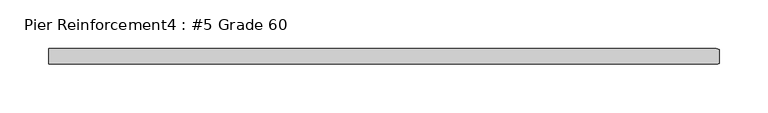
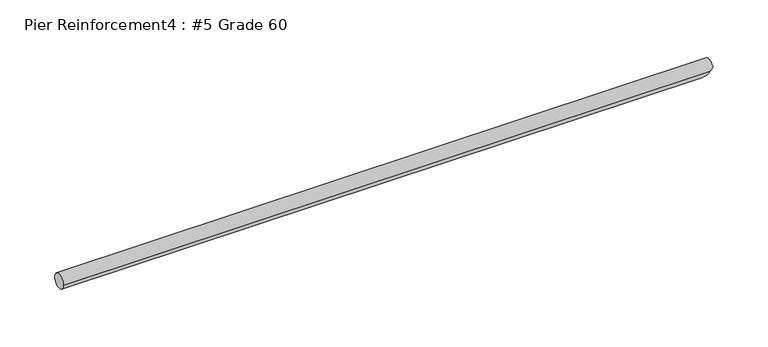
"""IFC4 building model written with IfcOpenShell, lengths in millimetres: proxy geometry, Pier Reinforcement4 : #5 Grade 60."""

import ifcopenshell
import ifcopenshell.guid

model = None  # the IFC model being written
_history = None  # IfcOwnerHistory: only IFC2X3 demands one
_inside = {}  # id of a spatial element -> (the spatial element, [elements in it])
_under = {}  # id of a project, library or spatial element -> (it, [spatial elements below it])
_declared = {}  # id of a project -> (the project, [libraries it declares])
_typed = {}  # id of a type object -> (the type object, [elements of that type])
_made_of = {}  # id of a material, layer set ... -> (it, [elements and type objects made of it])


def new_model(schema):
    """Start an empty IFC model of exactly this schema.

    Asked for "IFC4X3", IfcOpenShell would pick the latest addendum, in which some entities
    have other attributes; the version numbers below select the first issue.
    IFC2X3 requires an IfcOwnerHistory on every rooted entity: one is made here for all.
    """
    global model, _history
    if schema == "IFC4X3":
        model = ifcopenshell.file(schema_version=(4, 3, 0, 0))
    else:
        model = ifcopenshell.file(schema=schema)
    _inside.clear()
    _under.clear()
    _declared.clear()
    _typed.clear()
    _made_of.clear()
    _history = None
    if model.schema == "IFC2X3":
        org = make("IfcOrganization", Name="unknown")
        user = make(
            "IfcPersonAndOrganization",
            ThePerson=make("IfcPerson", FamilyName="unknown"),
            TheOrganization=org,
        )
        app = make(
            "IfcApplication",
            ApplicationDeveloper=org,
            Version="unknown",
            ApplicationFullName="unknown",
            ApplicationIdentifier="unknown",
        )
        _history = make(
            "IfcOwnerHistory",
            OwningUser=user,
            OwningApplication=app,
            ChangeAction="ADDED",
            CreationDate=0,
        )
    return model


def make(cls, **values):
    """One entity of the class cls with the attributes given. An attribute that is None is left unset."""
    return model.create_entity(
        cls, **{name: value for name, value in values.items() if value is not None}
    )


def rooted(cls, **values):
    """An entity with a GlobalId (a new one), such as an element, a storey or a relation."""
    return make(cls, GlobalId=ifcopenshell.guid.new(), OwnerHistory=_history, **values)


def si_unit(unit_type, name, prefix=None):
    """IfcSIUnit, for example si_unit("LENGTHUNIT", "METRE", prefix="MILLI")."""
    return make("IfcSIUnit", UnitType=unit_type, Prefix=prefix, Name=name)


def assignment(units):
    """IfcUnitAssignment: the units of a project."""
    return None if units is None else make("IfcUnitAssignment", Units=units)


def point(xyz):
    """IfcCartesianPoint."""
    return None if xyz is None else make("IfcCartesianPoint", Coordinates=xyz)


def direction(xyz):
    """IfcDirection."""
    return None if xyz is None else make("IfcDirection", DirectionRatios=xyz)


def frame(location, z_axis=None, x_axis=None):
    """IfcAxis2Placement3D, a coordinate frame: its origin and axes. An axis left out is left unset."""
    return make(
        "IfcAxis2Placement3D",
        Location=point(location),
        Axis=direction(z_axis),
        RefDirection=direction(x_axis),
    )


def origin():
    """The frame at (0, 0, 0) with its axes left unset."""
    return frame((0.0, 0.0, 0.0))


def place(relative_to, where):
    """IfcLocalPlacement: puts the frame where relative to a parent placement (None: the world)."""
    return make(
        "IfcLocalPlacement", PlacementRelTo=relative_to, RelativePlacement=where
    )


def context(
    kind, dimensions, precision=None, world=None, true_north=None, identifier=None
):
    """IfcGeometricRepresentationContext, for example the 3D "Model" context."""
    return make(
        "IfcGeometricRepresentationContext",
        ContextIdentifier=identifier,
        ContextType=kind,
        CoordinateSpaceDimension=dimensions,
        Precision=precision,
        WorldCoordinateSystem=world,
        TrueNorth=true_north,
    )


def project(units=None, contexts=None):
    """IfcProject with its units and contexts."""
    return rooted(
        "IfcProject",
        Name="project",
        RepresentationContexts=contexts,
        UnitsInContext=assignment(units),
    )


def spatial(cls, under=None, at=None, **own):
    """A site, building, storey or space (cls), placed at a placement, below another one or the project."""
    s = rooted(cls, ObjectPlacement=at, **own)
    if under is not None:
        _under.setdefault(under.id(), (under, []))[1].append(s)
    return s


def circle_curve(where, radius):
    """IfcCircle in the frame where."""
    return make("IfcCircle", Position=where, Radius=radius)


def ellipse_curve(where, semi_axis1, semi_axis2):
    """IfcEllipse in the frame where."""
    return make(
        "IfcEllipse", Position=where, SemiAxis1=semi_axis1, SemiAxis2=semi_axis2
    )


def shape(context_of_items, identifier, shape_type, items):
    """IfcShapeRepresentation: the items that make up one representation, for example the "Body"."""
    return make(
        "IfcShapeRepresentation",
        ContextOfItems=context_of_items,
        RepresentationIdentifier=identifier,
        RepresentationType=shape_type,
        Items=items,
    )


def source(mapping_origin, context_of_items, identifier, shape_type, items):
    """IfcRepresentationMap: a shape defined once, which mapped items show again and again."""
    return make(
        "IfcRepresentationMap",
        MappingOrigin=mapping_origin,
        MappedRepresentation=shape(context_of_items, identifier, shape_type, items),
    )


def transform(
    local_origin,
    x_axis=None,
    y_axis=None,
    z_axis=None,
    scale=None,
    scale2=None,
    scale3=None,
    uniform=True,
):
    """IfcCartesianTransformationOperator3D, or its non-uniform kind. x_axis, y_axis, z_axis: its Axis1, 2, 3."""
    if uniform:
        return make(
            "IfcCartesianTransformationOperator3D",
            Axis1=direction(x_axis),
            Axis2=direction(y_axis),
            LocalOrigin=point(local_origin),
            Scale=scale,
            Axis3=direction(z_axis),
        )
    return make(
        "IfcCartesianTransformationOperator3DnonUniform",
        Axis1=direction(x_axis),
        Axis2=direction(y_axis),
        LocalOrigin=point(local_origin),
        Scale=scale,
        Axis3=direction(z_axis),
        Scale2=scale2,
        Scale3=scale3,
    )


def mapped(mapping_source, mapping_target):
    """IfcMappedItem: shows the shape of a source again, moved by a transform."""
    return make(
        "IfcMappedItem", MappingSource=mapping_source, MappingTarget=mapping_target
    )


def made_of(thing, what):
    """Note that an element or type object is made of a material, layer set ...; save() writes the relation."""
    if what is not None:
        _made_of.setdefault(what.id(), (what, []))[1].append(thing)
    return thing


def element(
    cls,
    number,
    at=None,
    inside=None,
    cuts=None,
    type_object=None,
    material=None,
    context=None,
    identifier="Body",
    shape_type=None,
    held_by="IfcProductDefinitionShape",
    body=None,
    shapes=None,
    **own,
):
    """One element of the class cls, such as IfcWall. Its Tag is "e" and its number.

    at: its placement. inside: the storey or other place that contains it. cuts: it is an
    opening in that element (IfcRelVoidsElement). A single representation is given by context,
    identifier, shape_type and body (its items); several are given by shapes. held_by: the class
    of the entity that holds the representations. save() writes the other relations.
    """
    e = rooted(cls, Tag="e%d" % number, ObjectPlacement=at, **own)
    if body is not None:
        shapes = [shape(context, identifier, shape_type, body)]
    if shapes is not None:
        e.Representation = make(held_by, Representations=shapes)
    if inside is not None:
        _inside.setdefault(inside.id(), (inside, []))[1].append(e)
    if cuts is not None:
        rooted(
            "IfcRelVoidsElement", RelatingBuildingElement=cuts, RelatedOpeningElement=e
        )
    if type_object is not None:
        _typed.setdefault(type_object.id(), (type_object, []))[1].append(e)
    return made_of(e, material)


def aggregate(whole, parts):
    """IfcRelAggregates: a whole, such as a stair, and the parts it consists of."""
    return rooted("IfcRelAggregates", RelatingObject=whole, RelatedObjects=parts)


def save(model, path):
    """Write the relations noted so far, then the file.

    IfcRelAggregates (storeys below a building ...), IfcRelContainedInSpatialStructure (elements
    in a storey), IfcRelDefinesByType, IfcRelAssociatesMaterial and IfcRelDeclares: one each for
    every whole, place, type object, material and project.
    """
    for whole, parts in _under.values():
        aggregate(whole, parts)
    for where, things in _inside.values():
        rooted(
            "IfcRelContainedInSpatialStructure",
            RelatedElements=things,
            RelatingStructure=where,
        )
    for kind, things in _typed.values():
        rooted("IfcRelDefinesByType", RelatedObjects=things, RelatingType=kind)
    for what, things in _made_of.values():
        rooted("IfcRelAssociatesMaterial", RelatedObjects=things, RelatingMaterial=what)
    for by, libraries in _declared.values():
        rooted("IfcRelDeclares", RelatingContext=by, RelatedDefinitions=libraries)
    model.write(path)


def plane_surface(at):
    """IfcPlane: the flat surface through the origin of the frame at, square to its z axis."""
    return make("IfcPlane", Position=at)


def cylinder_surface(at, radius):
    """IfcCylindricalSurface: all points at the distance radius from the z axis of the frame at."""
    return make("IfcCylindricalSurface", Position=at, Radius=radius)


def advanced_brep(points, edges, surfaces, faces):
    """IfcAdvancedBrep: a solid bounded by faces that lie on surfaces and meet in shared edges.

    An edge is (start, end): straight between two places in points (the first is 0);
    or (start, end, curve); or (start, end, curve, False) where it runs against its curve.
    A face is (place in surfaces, loops), or (place, loops, False) where it looks against
    its surface's normal. A loop lists edges by number (the first is 1), with a minus sign
    where the edge is run from its end to its start. The first loop is the outer one.
    """
    corners = [point(p) for p in points]
    vertices = [make("IfcVertexPoint", VertexGeometry=c) for c in corners]
    made = []
    for start, end, *more in edges:
        made.append(
            make(
                "IfcEdgeCurve",
                EdgeStart=vertices[start],
                EdgeEnd=vertices[end],
                EdgeGeometry=more[0] if more else make("IfcPolyline", Points=[corners[start], corners[end]]),
                SameSense=more[1] if len(more) > 1 else True,
            )
        )
    hull = []
    for where, loops, *sense in faces:
        bounds = []
        for j, loop in enumerate(loops):
            ring = [make("IfcOrientedEdge", EdgeElement=made[abs(k) - 1], Orientation=k > 0) for k in loop]
            bounds.append(
                make(
                    "IfcFaceOuterBound" if j == 0 else "IfcFaceBound",
                    Bound=make("IfcEdgeLoop", EdgeList=ring),
                    Orientation=True,
                )
            )
        hull.append(make("IfcAdvancedFace", Bounds=bounds, FaceSurface=surfaces[where], SameSense=sense[0] if sense else True))
    return make("IfcAdvancedBrep", Outer=make("IfcClosedShell", CfsFaces=hull))


def pier_reinforcement4_5_grade_60_3385e020(model_context):
    return source(origin(), model_context, "Body", "AdvancedBrep", [
        advanced_brep(
        [(590233.9922365, -534089.3915452, -52.3875), (590233.9922365, -534103.941223, -52.3875), (589548.1922365, -534088.7288841, -55.5625), (589548.1922365, -534104.6038841, -55.5625), (590230.8172365, -534104.6038841, -55.5625), (590230.8172365, -534088.7288841, -55.5625), (590222.8797365, -534096.6663841, -63.5)],
        [
            (0, 1, circle_curve(frame((590233.9922365, -534096.6663841, -55.5625), z_axis=(1.0, 0.0, 0.0), x_axis=(0.0, -1.0, 0.0)), 7.9375)),
            (1, 0),
            (2, 3, circle_curve(frame((589548.1922365, -534096.6663841, -55.5625), z_axis=(-1.0, 0.0, 0.0), x_axis=(0.0, -1.0, 0.0)), 7.9375)),
            (3, 2, circle_curve(frame((589548.1922365, -534096.6663841, -55.5625), z_axis=(-1.0, 0.0, 0.0), x_axis=(0.0, -1.0, 0.0)), 7.9375)),
            (3, 4),
            (4, 1, ellipse_curve(frame((590230.8172365, -534096.6663841, -55.5625), z_axis=(-0.7071067811865462, 0.0, 0.7071067811865489), x_axis=(0.7071067811865487, 0.0, 0.7071067811865462)), 11.2253202, 7.9375)),
            (0, 5, ellipse_curve(frame((590230.8172365, -534096.6663841, -55.5625), z_axis=(-0.7071067811865462, 0.0, 0.7071067811865489), x_axis=(0.7071067811865487, 0.0, 0.7071067811865462)), 11.2253202, 7.9375)),
            (5, 2),
            (5, 6, ellipse_curve(frame((590230.8172365, -534096.6663841, -55.5625), z_axis=(-0.7071067811865462, 0.0, 0.7071067811865489), x_axis=(0.7071067811865487, 0.0, 0.7071067811865462)), 11.2253202, 7.9375)),
            (6, 4, ellipse_curve(frame((590230.8172365, -534096.6663841, -55.5625), z_axis=(-0.7071067811865462, 0.0, 0.7071067811865489), x_axis=(0.7071067811865487, 0.0, 0.7071067811865462)), 11.2253202, 7.9375)),
        ],
        [
            plane_surface(frame((590233.9922365, -534104.6038841, -55.5625), z_axis=(1.0, 0.0, 0.0), x_axis=(0.0, 0.0, -1.0))),
            plane_surface(frame((589548.1922365, -534104.6038841, -55.5625), z_axis=(-1.0, 0.0, 0.0), x_axis=(0.0, 0.0, 1.0))),
            cylinder_surface(frame((589548.1922365, -534096.6663841, -55.5625), z_axis=(1.0, 0.0, 0.0), x_axis=(0.0, -1.0, 0.0)), 7.9375),
            plane_surface(frame((590222.8797365, -534128.4163841, -63.5), z_axis=(0.7071067811865462, 0.0, -0.7071067811865489), x_axis=(0.0, 1.0, 0.0))),
        ],
        [
            (0, [[1, 2]]),
            (1, [[3, 4]]),
            (2, [[-4, 5, 6, -1, 7, 8]]),
            (2, [[-3, -8, 9, 10, -5]]),
            (3, [[-2, -6, -10, -9, -7]]),
        ],
    ),
    ])


if __name__ == "__main__":
    model = new_model("IFC4")
    model_context = context("Model", 3, world=origin())
    ifc_project = project(units=[si_unit("LENGTHUNIT", "METRE", prefix="MILLI")], contexts=[model_context])
    site = spatial("IfcSite", under=ifc_project)
    building = spatial("IfcBuilding", under=site)
    placement = place(None, origin())
    pier_reinforcement4_5_grade_60_shape = pier_reinforcement4_5_grade_60_3385e020(model_context)
    element("IfcBuildingElementProxy", 1, Name="Pier Reinforcement4 : #5 Grade 60", ObjectType="Pier Reinforcement4 : #5 Grade 60", at=placement, inside=building, context=model_context, shape_type="MappedRepresentation", body=[
        mapped(pier_reinforcement4_5_grade_60_shape, transform((0.0, 0.0, 0.0), x_axis=(1.0, 0.0, 0.0), y_axis=(0.0, 1.0, 0.0), z_axis=(0.0, 0.0, 1.0))),
    ])
    save(model, "model.ifc")

# Revit data of these elements
# Element 1 (IfcBuildingElementProxy, "Pier Reinforcement4 : #5 Grade 60")
#   Materials on its faces: "#4 GR. 60 REINF. @ 16\" O.C. EW."
# Materials
#   "#4 GR. 60 REINF. @ 16\" O.C. EW.": class "Generic", colour RGB 84 83 81, transparency 0, Cost = 0
